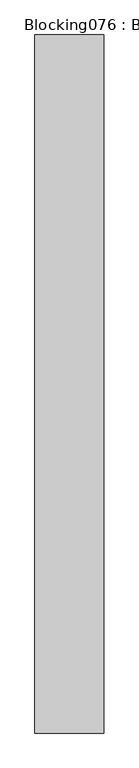
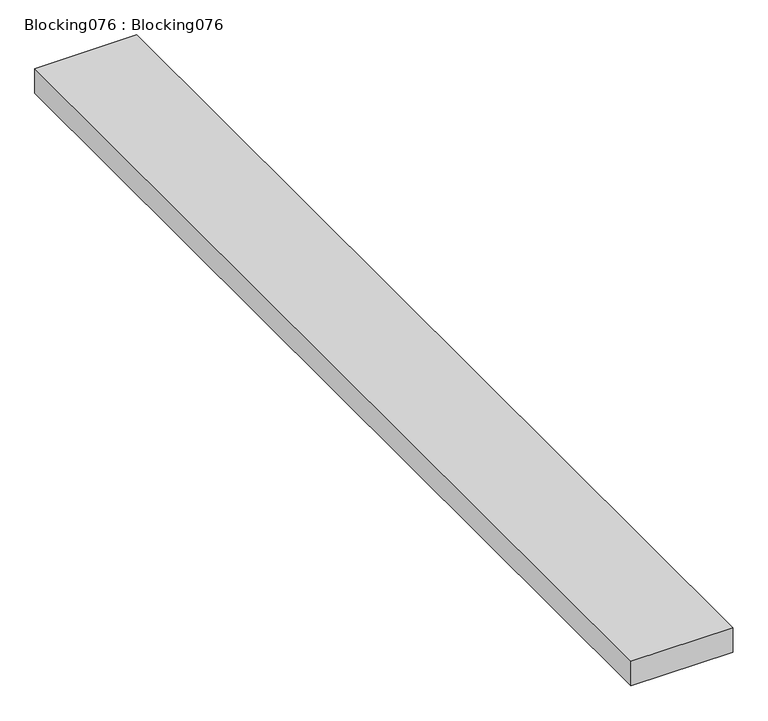
"""IFC4 building model written with IfcOpenShell, lengths in millimetres: proxy geometry, Blocking076 : Blocking076."""

from ifc_helpers import new_model, si_unit, frame, origin, place, context, project, spatial, polyline, outline, extrude, source, transform, mapped, element, save


def blocking076_blocking076_732f58c6(model_context):
    return source(origin(), model_context, "Body", "SweptSolid", [
        extrude(outline(polyline([(-2567.3737014, -1052.8906574), (-2764.2237014, -1052.8906574), (-2764.2237014, 947.1093426), (-2567.3737014, 947.1093426), (-2567.3737014, -1052.8906574)])), frame((0.0, 0.0, 40182.546), z_axis=(0.0, 0.0, 1.0), x_axis=(1.0, 0.0, 0.0)), (0.0, 0.0, 1.0), 50.8),
    ])


if __name__ == "__main__":
    model = new_model("IFC4")
    model_context = context("Model", 3, world=origin())
    ifc_project = project(units=[si_unit("LENGTHUNIT", "METRE", prefix="MILLI")], contexts=[model_context])
    site = spatial("IfcSite", under=ifc_project)
    building = spatial("IfcBuilding", under=site)
    placement = place(None, origin())
    blocking076_blocking076_shape = blocking076_blocking076_732f58c6(model_context)
    element("IfcBuildingElementProxy", 1, Name="Blocking076 : Blocking076", ObjectType="Blocking076 : Blocking076", at=placement, inside=building, context=model_context, shape_type="MappedRepresentation", body=[
        mapped(blocking076_blocking076_shape, transform((0.0, 0.0, 0.0), x_axis=(1.0, 0.0, 0.0), y_axis=(0.0, 1.0, 0.0), z_axis=(0.0, 0.0, 1.0))),
    ])
    save(model, "model.ifc")

# Revit data of these elements
# Type "Blocking076 : Blocking076"
#   NameOverride = "Blocking076"
# Element 1 (IfcBuildingElementProxy, "Blocking076 : Blocking076")
#   Materials on its faces: "WOOD BLOCKING AS REQUIRED"
# Materials
#   "WOOD BLOCKING AS REQUIRED": class "Unassigned", colour RGB 166 124 85, transparency 0, Cost = 0
